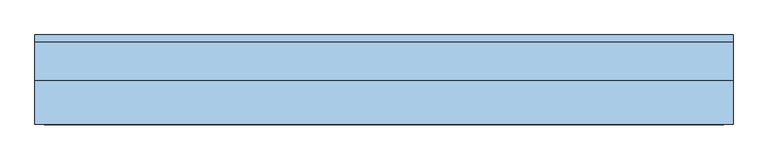
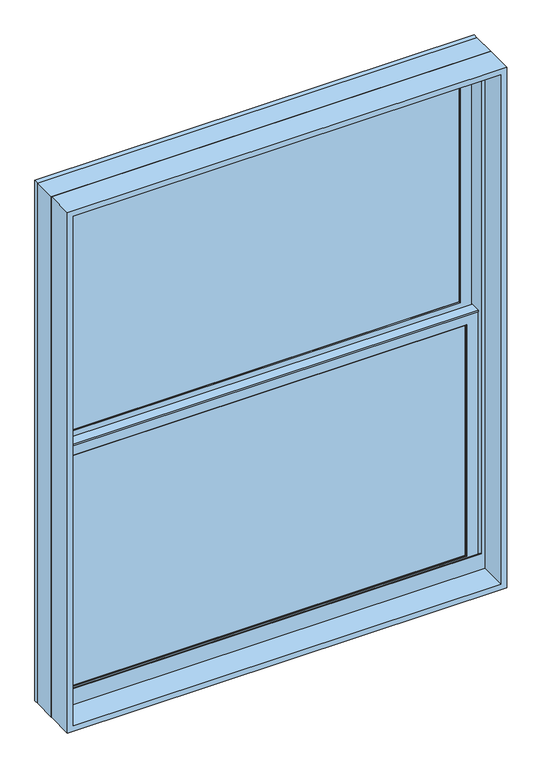
"""IFC4 building model written with IfcOpenShell, lengths in millimetres: window geometry, Window-Double_Hung-Marvin-Essential : ESDH4050."""

from ifc_helpers import new_model, si_unit, frame, origin, place, context, project, spatial, polyline, outline, extrude, faceted_brep, source, transform, mapped, element, save


def window_9aae5a61(model_context):
    return source(origin(), model_context, "Body", "SolidModel", [
        extrude(outline(polyline([(191.5583333, 20.6375), (191.5583333, 15.875), (172.5083333, 15.875), (172.5083333, 20.6375), (191.5583333, 20.6375)])), frame((0.0, 0.0, 984.25), z_axis=(0.0, 0.0, 1.0), x_axis=(1.0, 0.0, 0.0)), (0.0, 0.0, 1.0), 679.45),
        extrude(outline(polyline([(-172.5083333, 20.6375), (-172.5083333, 15.875), (-191.5583333, 15.875), (-191.5583333, 20.6375), (-172.5083333, 20.6375)])), frame((0.0, 0.0, 984.25), z_axis=(0.0, 0.0, 1.0), x_axis=(1.0, 0.0, 0.0)), (0.0, 0.0, 1.0), 679.45),
        extrude(outline(polyline([(546.1, 20.6375), (546.1, 15.875), (-546.1, 15.875), (-546.1, 20.6375), (546.1, 20.6375)])), frame((0.0, 0.0, 1314.45), z_axis=(0.0, 0.0, 1.0), x_axis=(1.0, 0.0, 0.0)), (0.0, 0.0, 1.0), 19.05),
        extrude(outline(polyline([(-191.5583333, 46.83125), (-191.5583333, 51.59375), (-172.5083333, 51.59375), (-172.5083333, 46.83125), (-191.5583333, 46.83125)])), frame((0.0, 0.0, 1701.8), z_axis=(0.0, 0.0, 1.0), x_axis=(1.0, 0.0, 0.0)), (0.0, 0.0, 1.0), 679.45),
        extrude(outline(polyline([(172.5083333, 46.83125), (172.5083333, 51.59375), (191.5583333, 51.59375), (191.5583333, 46.83125), (172.5083333, 46.83125)])), frame((0.0, 0.0, 1701.8), z_axis=(0.0, 0.0, 1.0), x_axis=(1.0, 0.0, 0.0)), (0.0, 0.0, 1.0), 679.45),
        extrude(outline(polyline([(-546.1, 46.83125), (-546.1, 51.59375), (546.1, 51.59375), (546.1, 46.83125), (-546.1, 46.83125)])), frame((0.0, 0.0, 2032.0), z_axis=(0.0, 0.0, 1.0), x_axis=(1.0, 0.0, 0.0)), (0.0, 0.0, 1.0), 19.05),
        extrude(outline(polyline([(191.5583333, 20.6375), (172.5083333, 20.6375), (172.5083333, 25.4), (191.5583333, 25.4), (191.5583333, 20.6375)])), frame((0.0, 0.0, 984.25), z_axis=(0.0, 0.0, 1.0), x_axis=(1.0, 0.0, 0.0)), (0.0, 0.0, 1.0), 679.45),
        extrude(outline(polyline([(-172.5083333, 20.6375), (-191.5583333, 20.6375), (-191.5583333, 25.4), (-172.5083333, 25.4), (-172.5083333, 20.6375)])), frame((0.0, 0.0, 984.25), z_axis=(0.0, 0.0, 1.0), x_axis=(1.0, 0.0, 0.0)), (0.0, 0.0, 1.0), 679.45),
        extrude(outline(polyline([(546.1, 20.6375), (-546.1, 20.6375), (-546.1, 25.4), (546.1, 25.4), (546.1, 20.6375)])), frame((0.0, 0.0, 1314.45), z_axis=(0.0, 0.0, 1.0), x_axis=(1.0, 0.0, 0.0)), (0.0, 0.0, 1.0), 19.05),
        extrude(outline(polyline([(-191.5583333, 56.35625), (-172.5083333, 56.35625), (-172.5083333, 51.59375), (-191.5583333, 51.59375), (-191.5583333, 56.35625)])), frame((0.0, 0.0, 1701.8), z_axis=(0.0, 0.0, 1.0), x_axis=(1.0, 0.0, 0.0)), (0.0, 0.0, 1.0), 679.45),
        extrude(outline(polyline([(172.5083333, 56.35625), (191.5583333, 56.35625), (191.5583333, 51.59375), (172.5083333, 51.59375), (172.5083333, 56.35625)])), frame((0.0, 0.0, 1701.8), z_axis=(0.0, 0.0, 1.0), x_axis=(1.0, 0.0, 0.0)), (0.0, 0.0, 1.0), 679.45),
        extrude(outline(polyline([(-546.1, 56.35625), (546.1, 56.35625), (546.1, 51.59375), (-546.1, 51.59375), (-546.1, 56.35625)])), frame((0.0, 0.0, 2032.0), z_axis=(0.0, 0.0, 1.0), x_axis=(1.0, 0.0, 0.0)), (0.0, 0.0, 1.0), 19.05),
        faceted_brep([(-573.0875, 5.6780605, 1693.7351748), (-573.0875, 5.6780605, 1689.1), (573.0875, 5.6780605, 1689.1), (573.0875, 5.6780605, 1693.7351748), (-573.0875, 34.8118605, 1693.7351748), (573.0875, 34.8118605, 1693.7351748), (573.0875, 34.8118605, 1689.1), (-573.0875, 34.8118605, 1689.1), (-573.0875, 30.1625, 1689.1), (-573.0875, 30.1625, 957.2625), (-573.0875, 8.9241104, 957.2625), (-573.0875, 8.9241104, 1689.1), (573.0875, 8.9241104, 1689.1), (573.0875, 30.1625, 1689.1), (573.0875, 8.9241104, 957.2625), (573.0875, 30.1625, 957.2625), (-557.2034752, 11.90625, 1674.8034752), (-557.2034752, 30.1625, 1674.8034752), (557.2034752, 30.1625, 1674.8034752), (557.2034752, 11.90625, 1674.8034752), (-540.54375, 10.4662439, 1658.14375), (-540.54375, 11.90625, 1658.14375), (540.54375, 11.90625, 1658.14375), (540.54375, 10.4662439, 1658.14375), (542.0858834, 8.9241104, 1659.6858834), (-542.0858834, 8.9241104, 1659.6858834), (557.2034752, 30.1625, 973.1465248), (557.2034752, 11.90625, 973.1465248), (540.54375, 11.90625, 989.80625), (540.54375, 10.4662439, 989.80625), (542.0858834, 8.9241104, 988.2641166), (-557.2034752, 30.1625, 973.1465248), (-557.2034752, 11.90625, 973.1465248), (-540.54375, 11.90625, 989.80625), (-540.54375, 10.4662439, 989.80625), (-542.0858834, 8.9241104, 988.2641166)], [[[0, 1, 2, 3]], [[4, 5, 6, 7]], [[1, 0, 4, 7, 8, 9, 10, 11]], [[2, 1, 11, 12]], [[7, 6, 13, 8]], [[3, 2, 12, 14, 15, 13, 6, 5]], [[0, 3, 5, 4]], [[16, 17, 18, 19]], [[20, 21, 22, 23]], [[20, 23, 24, 25]], [[19, 18, 26, 27]], [[23, 22, 28, 29]], [[24, 23, 29, 30]], [[27, 26, 31, 32]], [[29, 28, 33, 34]], [[30, 29, 34, 35]], [[15, 14, 10, 9]], [[15, 9, 8, 13], [18, 17, 31, 26]], [[17, 16, 32, 31]], [[16, 19, 27, 32], [22, 21, 33, 28]], [[21, 20, 34, 33]], [[20, 25, 35, 34]], [[10, 14, 12, 11], [25, 24, 30, 35]]]),
        extrude(outline(polyline([(38.5955581, 1674.8125), (33.5778968, 1674.8125), (33.5778968, 1676.4), (39.9405976, 1676.4), (39.9405976, 1674.8125), (61.515625, 1674.8125), (47.6307501, 1671.4975159), (38.5955581, 1671.4975159), (38.5955581, 1674.8125)])), frame((-573.0875, 0.0, 0.0), z_axis=(1.0, 0.0, 0.0), x_axis=(0.0, 1.0, 0.0)), (0.0, 0.0, 1.0), 1146.175),
        faceted_brep([(603.25, 0.0, 927.1), (603.25, 0.0, 2438.4), (-603.25, 0.0, 2438.4), (-603.25, 0.0, 927.1), (577.05625, 0.0, 988.21875), (-577.05625, 0.0, 988.21875), (-577.05625, 0.0, 2412.20625), (577.05625, 0.0, 2412.20625), (577.05625, 3.96875, 927.1), (-577.05625, 3.96875, 927.1), (-577.05625, 3.96875, 988.21875), (577.05625, 3.96875, 988.21875), (-603.25, 65.6828125, 927.1), (-577.05625, 65.6828125, 927.1), (577.05625, 65.6828125, 927.1), (603.25, 65.6828125, 927.1), (-603.25, 65.6828125, 2438.4), (603.25, 65.6828125, 2438.4), (577.05625, 65.6828125, 2412.20625), (-577.05625, 65.6828125, 2412.20625)], [[[0, 1, 2, 3], [4, 5, 6, 7]], [[8, 9, 10, 11]], [[5, 4, 11, 10]], [[0, 3, 12, 13, 9, 8, 14, 15]], [[13, 12, 16, 17, 15, 14, 18, 19]], [[13, 19, 6, 5, 10, 9]], [[7, 6, 19, 18]], [[18, 14, 8, 11, 4, 7]], [[1, 0, 15, 17]], [[2, 1, 17, 16]], [[3, 2, 16, 12]]]),
        faceted_brep([(577.05625, 30.1625, 1682.75), (575.46875, 30.1625, 1682.75), (575.46875, 30.1625, 951.4544613), (577.05625, 30.1625, 951.4544613), (-575.46875, 30.1625, 1682.75), (-577.05625, 30.1625, 1682.75), (-577.05625, 30.1625, 951.4544613), (-575.46875, 30.1625, 951.4544613), (575.46875, 63.5, 1682.75), (577.05625, 63.5, 1682.75), (577.05625, 63.5, 944.9743077), (575.46875, 63.5, 944.9743077), (-577.05625, 63.5, 1682.75), (-575.46875, 63.5, 1682.75), (-575.46875, 63.5, 944.9743077), (-577.05625, 63.5, 944.9743077), (588.3108932, 3.96875, 956.5460105), (588.3108932, 3.96875, 927.1), (588.3108932, 65.6828125, 927.1), (588.3108932, 65.6828125, 944.550012), (-588.3108932, 3.96875, 927.1), (-588.3108932, 3.96875, 956.5460105), (-588.3108932, 65.6828125, 944.550012), (-588.3108932, 65.6828125, 927.1), (588.3108932, 78.58125, 942.0428097), (-588.3108932, 78.58125, 942.0428097), (-586.2971252, 68.2348864, 944.0539391), (-568.33135, 68.2348864, 944.0539391), (-568.33135, 65.6828125, 944.550012), (568.33135, 65.6828125, 944.550012), (568.33135, 68.2348864, 944.0539391), (586.2971252, 68.2348864, 944.0539391), (-603.25, 65.6828125, 927.1), (-603.25, 78.5948249, 927.1), (603.25, 78.5948249, 927.1), (603.25, 65.6828125, 927.1), (-603.25, 78.58125, 2438.4), (603.25, 78.58125, 2438.4), (588.3108932, 78.58125, 2423.4608932), (-588.3108932, 78.58125, 2423.4608932), (-603.25, 65.6828125, 2438.4), (-586.2971252, 68.2348864, 2421.4471252), (586.2971252, 68.2348864, 2421.4471252), (568.33135, 68.2348864, 2403.48135), (-568.33135, 68.2348864, 2403.48135), (-568.33135, 65.6828125, 2403.48135), (568.33135, 65.6828125, 2403.48135), (603.25, 65.6828125, 2438.4)], [[[0, 1, 2, 3]], [[4, 5, 6, 7]], [[8, 9, 10, 11]], [[12, 13, 14, 15]], [[1, 8, 11, 2]], [[9, 0, 3, 10]], [[1, 0, 9, 8]], [[5, 4, 13, 12]], [[5, 12, 15, 6]], [[13, 4, 7, 14]], [[16, 17, 18, 19]], [[20, 21, 22, 23]], [[24, 25, 26, 27, 28, 22, 21, 16, 19, 29, 30, 31], [3, 2, 11, 10], [7, 6, 15, 14]], [[17, 16, 21, 20]], [[17, 20, 23, 32, 33, 34, 35, 18]], [[34, 33, 36, 37], [25, 24, 38, 39]], [[33, 32, 40, 36]], [[39, 41, 26, 25]], [[41, 42, 31, 30, 43, 44, 27, 26]], [[44, 45, 28, 27]], [[40, 32, 23, 22, 28, 45, 46, 29, 19, 18, 35, 47]], [[36, 40, 47, 37]], [[39, 38, 42, 41]], [[44, 43, 46, 45]], [[34, 37, 47, 35]], [[42, 38, 24, 31]], [[46, 43, 30, 29]]]),
        extrude(outline(polyline([(553.24375, 11.90625), (-553.24375, 11.90625), (-553.24375, 15.08125), (553.24375, 15.08125), (553.24375, 11.90625)])), frame((0.0, 0.0, 977.10625), z_axis=(0.0, 0.0, 1.0), x_axis=(1.0, 0.0, 0.0)), (0.0, 0.0, 1.0), 693.7375),
        extrude(outline(polyline([(553.24375, 42.8625), (-553.24375, 42.8625), (-553.24375, 46.0375), (553.24375, 46.0375), (553.24375, 42.8625)])), frame((0.0, 0.0, 1694.65625), z_axis=(0.0, 0.0, 1.0), x_axis=(1.0, 0.0, 0.0)), (0.0, 0.0, 1.0), 693.7375),
        faceted_brep([(-540.54375, 31.194477, 1658.14375), (-542.0858834, 32.7366104, 1659.6858834), (542.0858834, 32.7366104, 1659.6858834), (540.54375, 31.194477, 1658.14375), (-540.54375, 30.1625, 1658.14375), (540.54375, 30.1625, 1658.14375), (-573.0875, 32.7366104, 1690.6875), (-573.0875, 30.1625, 1690.6875), (573.0875, 30.1625, 1690.6875), (573.0875, 32.7366104, 1690.6875), (542.0858834, 32.7366104, 988.2641166), (540.54375, 31.194477, 989.80625), (540.54375, 30.1625, 989.80625), (573.0875, 30.1625, 957.2625), (573.0875, 32.7366104, 957.2625), (-542.0858834, 32.7366104, 988.2641166), (-540.54375, 31.194477, 989.80625), (-540.54375, 30.1625, 989.80625), (-573.0875, 30.1625, 957.2625), (-573.0875, 32.7366104, 957.2625)], [[[0, 1, 2, 3]], [[4, 0, 3, 5]], [[6, 7, 8, 9]], [[3, 2, 10, 11]], [[5, 3, 11, 12]], [[9, 8, 13, 14]], [[11, 10, 15, 16]], [[12, 11, 16, 17]], [[14, 13, 18, 19]], [[9, 14, 19, 6], [1, 15, 10, 2]], [[16, 15, 1, 0]], [[17, 16, 0, 4]], [[7, 18, 13, 8], [5, 12, 17, 4]], [[19, 18, 7, 6]]]),
        faceted_brep([(-557.2034752, 42.8625, 2392.3534752), (-557.2034752, 61.11875, 2392.3534752), (557.2034752, 61.11875, 2392.3534752), (557.2034752, 42.8625, 2392.3534752), (-540.54375, 41.4224939, 2375.69375), (-540.54375, 42.8625, 2375.69375), (540.54375, 42.8625, 2375.69375), (540.54375, 41.4224939, 2375.69375), (-542.0858834, 39.8803604, 2377.2358834), (542.0858834, 39.8803604, 2377.2358834), (-573.0875, 61.11875, 2408.2375), (-573.0875, 39.8803604, 2408.2375), (573.0875, 39.8803604, 2408.2375), (573.0875, 61.11875, 2408.2375), (557.2034752, 61.11875, 1690.6965248), (557.2034752, 42.8625, 1690.6965248), (540.54375, 42.8625, 1707.35625), (540.54375, 41.4224939, 1707.35625), (542.0858834, 39.8803604, 1705.8141166), (573.0875, 39.8803604, 1674.8125), (573.0875, 61.11875, 1674.8125), (-557.2034752, 61.11875, 1690.6965248), (-557.2034752, 42.8625, 1690.6965248), (-540.54375, 42.8625, 1707.35625), (-540.54375, 41.4224939, 1707.35625), (-542.0858834, 39.8803604, 1705.8141166), (-573.0875, 39.8803604, 1674.8125), (-573.0875, 61.11875, 1674.8125)], [[[0, 1, 2, 3]], [[4, 5, 6, 7]], [[8, 4, 7, 9]], [[10, 11, 12, 13]], [[3, 2, 14, 15]], [[7, 6, 16, 17]], [[9, 7, 17, 18]], [[13, 12, 19, 20]], [[15, 14, 21, 22]], [[17, 16, 23, 24]], [[18, 17, 24, 25]], [[20, 19, 26, 27]], [[13, 20, 27, 10], [1, 21, 14, 2]], [[22, 21, 1, 0]], [[3, 15, 22, 0], [5, 23, 16, 6]], [[24, 23, 5, 4]], [[25, 24, 4, 8]], [[11, 26, 19, 12], [9, 18, 25, 8]], [[27, 26, 11, 10]]]),
        faceted_brep([(-573.0875, 61.11875, 1674.8125), (-573.0875, 63.6928604, 1674.8125), (573.0875, 63.6928604, 1674.8125), (573.0875, 61.11875, 1674.8125), (-540.54375, 62.150727, 1707.35625), (-540.54375, 61.11875, 1707.35625), (540.54375, 61.11875, 1707.35625), (540.54375, 62.150727, 1707.35625), (-542.0858834, 63.6928604, 1705.8141166), (542.0858834, 63.6928604, 1705.8141166), (573.0875, 63.6928604, 2408.2375), (573.0875, 61.11875, 2408.2375), (540.54375, 61.11875, 2375.69375), (540.54375, 62.150727, 2375.69375), (542.0858834, 63.6928604, 2377.2358834), (-573.0875, 63.6928604, 2408.2375), (-573.0875, 61.11875, 2408.2375), (-540.54375, 61.11875, 2375.69375), (-540.54375, 62.150727, 2375.69375), (-542.0858834, 63.6928604, 2377.2358834)], [[[0, 1, 2, 3]], [[4, 5, 6, 7]], [[8, 4, 7, 9]], [[3, 2, 10, 11]], [[7, 6, 12, 13]], [[9, 7, 13, 14]], [[11, 10, 15, 16]], [[13, 12, 17, 18]], [[14, 13, 18, 19]], [[16, 15, 1, 0]], [[3, 11, 16, 0], [5, 17, 12, 6]], [[18, 17, 5, 4]], [[19, 18, 4, 8]], [[1, 15, 10, 2], [9, 14, 19, 8]]]),
        extrude(outline(polyline([(553.24375, 26.19375), (-553.24375, 26.19375), (-553.24375, 30.1625), (553.24375, 30.1625), (553.24375, 26.19375)])), frame((0.0, 0.0, 977.10625), z_axis=(0.0, 0.0, 1.0), x_axis=(1.0, 0.0, 0.0)), (0.0, 0.0, 1.0), 693.7375),
        extrude(outline(polyline([(553.24375, 57.15), (-553.24375, 57.15), (-553.24375, 61.11875), (553.24375, 61.11875), (553.24375, 57.15)])), frame((0.0, 0.0, 1694.65625), z_axis=(0.0, 0.0, 1.0), x_axis=(1.0, 0.0, 0.0)), (0.0, 0.0, 1.0), 693.7375),
        extrude(outline(polyline([(2438.4, 603.25), (2438.4, -603.25), (927.1, -603.25), (927.1, 603.25), (2438.4, 603.25)]), holes=[polyline([(2422.525, 587.375), (942.975, 587.375), (942.975, -587.375), (2422.525, -587.375), (2422.525, 587.375)])]), frame((0.0, -76.2, 0.0), z_axis=(0.0, 1.0, 0.0), x_axis=(0.0, 0.0, 1.0)), (0.0, 0.0, 1.0), 75.40625),
    ])


if __name__ == "__main__":
    model = new_model("IFC4")
    model_context = context("Model", 3, world=origin())
    ifc_project = project(units=[si_unit("LENGTHUNIT", "METRE", prefix="MILLI")], contexts=[model_context])
    site = spatial("IfcSite", under=ifc_project)
    building = spatial("IfcBuilding", under=site)
    placement = place(None, origin())
    window_shape = window_9aae5a61(model_context)
    element("IfcWindow", 1, ObjectType="Window-Double_Hung-Marvin-Essential : ESDH4050", at=placement, inside=building, context=model_context, shape_type="MappedRepresentation", body=[
        mapped(window_shape, transform((0.0, 0.0, 0.0), x_axis=(1.0, 0.0, 0.0), y_axis=(0.0, 1.0, 0.0), z_axis=(0.0, 0.0, 1.0))),
    ])
    save(model, "model.ifc")

# Revit data of these elements
# Type "Window-Double_Hung-Marvin-Essential : ESDH4050"
#   Type Mark = "67"
#   Window Type = "Essential Double Hung"
#   Product data url = "https://bimobject.com/marvin-windows-and-doors/product/marvin-dhwau"
#   Product Guid = "c4a96547-874c-4385-91dc-a058adc19d98"
#   Frame = "All Ultrex"
#   Egress Window = "Yes"
#   URL = "www.marvin.com"
#   Model = "ESDH4050"
#   Manufacturer = "Marvin Windows and Doors"
#   Label Egress = "EGRESS WDW"
#   Glass Type = "IG Low E II with Argon"
#   Design Pressure = "DP40"
#   Description = "4860 DBHG"
#   Analytic Construction = "<None>"
#   Prairie Corner Width = 0' - 4"
#   Prairie Corner Height = 0' - 4"
#   Egress Width = 3' - 8 9/16"
#   Egress Height = 2' - 1 27/128"
#   Rough Width = 4' - 0"
#   Rough Height = 5' - 0"
#   Nominal Width = 4' - 0"
#   Nominal Height = 5' - 0"
#   Inset to Installation Flange [instance default] = 0' - 1"
#   Height = 4' - 11 1/2"
#   Egress Area = 7.80182 SF
#   Default Head Height = 8' - 0"
#   Width = 3' - 11 1/2"
#   Daylight Area = 15.5545 SF
#   DLO Width = 3' - 6 9/16"
#   DLO Height = 2' - 2 5/16"
#   Muntins Top Sash = yes
#   Lites Wide Top Sash = 3
#   Lites Wide Bottom Sash = 3
#   Lites High Top Sash = 2
#   Lites High Bottom Sash = 2
#   Lite Cut Prairie 9 = no
#   Lite Cut HV Grid = yes
#   Muntins Bottom Sash = yes
#   Label Visibility = no
#   Jamb Extension Visibility = yes
#   Edition number = 1
#   Interior Material = Ultrex-Marvin-Stonewhite
#   Glazing Material = Glass-Marvin-IG Low E II with Argon
#   Cladding Material = Ultrex-Marvin-Pebblegray
#   Wall Closure = (empty or 0)
#   Assembly Code = ""
# Element 1 (IfcWindow, "Window-Double_Hung-Marvin-Essential : ESDH4050")
#   Materials on its faces: "Ultrex-Marvin-Pebblegray", "Ultrex-Marvin-Stonewhite", "Glass-Marvin-IG Low E II with Argon"
# Materials
#   "Ultrex-Marvin-Stonewhite": class "Paint", colour RGB 250 251 245, transparency 0
#   "Glass-Marvin-IG Low E II with Argon": class "Glass", colour RGB 0 128 192, transparency 0.85
#   "Ultrex-Marvin-Pebblegray": class "Paint", colour RGB 189 185 173, transparency 0
